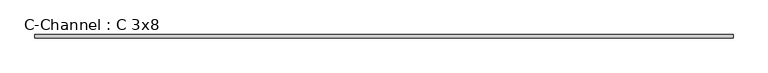
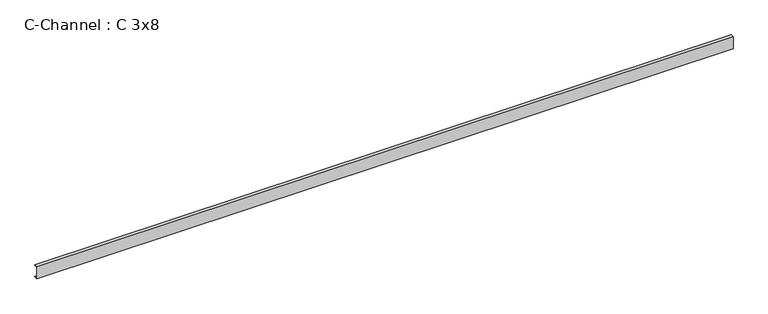
"""IFC4 building model written with IfcOpenShell, lengths in millimetres: beam geometry, C-Channel : C 3x8."""

from ifc_helpers import new_model, si_unit, point, frame, frame_2d, origin, place, context, project, spatial, polyline, circle_curve, trimmed, segment, composite_curve, outline, extrude, source, transform, mapped, element, save


def c_channel_c_3x8_0f36229c(model_context):
    return source(origin(), model_context, "Body", "SweptSolid", [
        extrude(outline(composite_curve([segment(polyline([(-13.5128, 101.6), (44.9072, 101.6)]), True, "CONTINUOUS"), segment(trimmed(circle_curve(frame_2d((35.6108, 101.6)), 9.2964), [point((44.9072, 101.6))], [point((35.6108, 92.3036))], False, "CARTESIAN"), True, "CONTINUOUS"), segment(polyline([(35.6108, 92.3036), (-2.8702, 86.2088084), (-2.8702, -86.2088084), (35.6108, -92.3036)]), True, "CONTINUOUS"), segment(trimmed(circle_curve(frame_2d((35.6108, -101.6)), 9.2964), [point((35.6108, -92.3036))], [point((44.9072, -101.6))], False, "CARTESIAN"), True, "CONTINUOUS"), segment(polyline([(44.9072, -101.6), (-13.5128, -101.6), (-13.5128, 101.6)]), True, "CONTINUOUS")], self_intersect=False)), frame((-12252.325, 0.0, 0.0), z_axis=(1.0, 0.0, 0.0), x_axis=(0.0, 1.0, 0.0)), (0.0, 0.0, 1.0), 11468.1),
    ])


if __name__ == "__main__":
    model = new_model("IFC4")
    model_context = context("Model", 3, world=origin())
    ifc_project = project(units=[si_unit("LENGTHUNIT", "METRE", prefix="MILLI")], contexts=[model_context])
    site = spatial("IfcSite", under=ifc_project)
    building = spatial("IfcBuilding", under=site)
    placement = place(None, origin())
    c_channel_c_3x8_shape = c_channel_c_3x8_0f36229c(model_context)
    element("IfcBeam", 1, ObjectType="C-Channel : C 3x8", at=placement, inside=building, context=model_context, shape_type="MappedRepresentation", body=[
        mapped(c_channel_c_3x8_shape, transform((0.0, 0.0, 0.0), x_axis=(1.0, 0.0, 0.0), y_axis=(0.0, 1.0, 0.0), z_axis=(0.0, 0.0, 1.0))),
    ])
    save(model, "model.ifc")

# Revit data of these elements
# Type "C-Channel : C 3x8"
#   Assembly Code = "B10"
#   W = 14.7
#   Length [instance default] = 5' - 0"
#   bf = 0' - 2.3"
#   d = 0' - 8"
#   tf = 0' - 0.366"
#   tw = 0' - 0.419"
#   x = 0' - 0.532"
#   A = 0.0300694 SF
#   Structural Material [instance default] = Steel ASTM A36
# Element 1 (IfcBeam, "C-Channel : C 3x8")
#   Structural Material = Steel ASTM A992
#   Materials on its faces: "Steel ASTM A992"
# Materials
#   "Steel ASTM A36": class "Metal", colour RGB 199 199 199, transparency 0, Description = "Structural steel, ASTM A36 Grade B, mill finish", Cost = 0
#   "Steel ASTM A992": class "Metal", colour RGB 189 187 185, transparency 0, Description = "Structural steel 50ksi", Cost = 0
